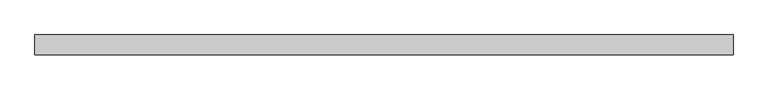
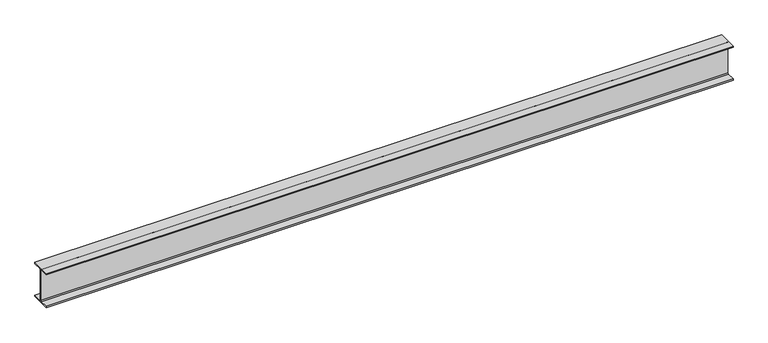
"""IFC4 building model written with IfcOpenShell, lengths in millimetres: beam geometry, Old_Steel Beam_H-KSD3502 : H_SB_ASB_H-350×175x7x11."""

import ifcopenshell
import ifcopenshell.guid

model = None  # the IFC model being written
_history = None  # IfcOwnerHistory: only IFC2X3 demands one
_inside = {}  # id of a spatial element -> (the spatial element, [elements in it])
_under = {}  # id of a project, library or spatial element -> (it, [spatial elements below it])
_declared = {}  # id of a project -> (the project, [libraries it declares])
_typed = {}  # id of a type object -> (the type object, [elements of that type])
_made_of = {}  # id of a material, layer set ... -> (it, [elements and type objects made of it])


def new_model(schema):
    """Start an empty IFC model of exactly this schema.

    Asked for "IFC4X3", IfcOpenShell would pick the latest addendum, in which some entities
    have other attributes; the version numbers below select the first issue.
    IFC2X3 requires an IfcOwnerHistory on every rooted entity: one is made here for all.
    """
    global model, _history
    if schema == "IFC4X3":
        model = ifcopenshell.file(schema_version=(4, 3, 0, 0))
    else:
        model = ifcopenshell.file(schema=schema)
    _inside.clear()
    _under.clear()
    _declared.clear()
    _typed.clear()
    _made_of.clear()
    _history = None
    if model.schema == "IFC2X3":
        org = make("IfcOrganization", Name="unknown")
        user = make(
            "IfcPersonAndOrganization",
            ThePerson=make("IfcPerson", FamilyName="unknown"),
            TheOrganization=org,
        )
        app = make(
            "IfcApplication",
            ApplicationDeveloper=org,
            Version="unknown",
            ApplicationFullName="unknown",
            ApplicationIdentifier="unknown",
        )
        _history = make(
            "IfcOwnerHistory",
            OwningUser=user,
            OwningApplication=app,
            ChangeAction="ADDED",
            CreationDate=0,
        )
    return model


def make(cls, **values):
    """One entity of the class cls with the attributes given. An attribute that is None is left unset."""
    return model.create_entity(
        cls, **{name: value for name, value in values.items() if value is not None}
    )


def rooted(cls, **values):
    """An entity with a GlobalId (a new one), such as an element, a storey or a relation."""
    return make(cls, GlobalId=ifcopenshell.guid.new(), OwnerHistory=_history, **values)


def si_unit(unit_type, name, prefix=None):
    """IfcSIUnit, for example si_unit("LENGTHUNIT", "METRE", prefix="MILLI")."""
    return make("IfcSIUnit", UnitType=unit_type, Prefix=prefix, Name=name)


def assignment(units):
    """IfcUnitAssignment: the units of a project."""
    return None if units is None else make("IfcUnitAssignment", Units=units)


def point(xyz):
    """IfcCartesianPoint."""
    return None if xyz is None else make("IfcCartesianPoint", Coordinates=xyz)


def direction(xyz):
    """IfcDirection."""
    return None if xyz is None else make("IfcDirection", DirectionRatios=xyz)


def frame(location, z_axis=None, x_axis=None):
    """IfcAxis2Placement3D, a coordinate frame: its origin and axes. An axis left out is left unset."""
    return make(
        "IfcAxis2Placement3D",
        Location=point(location),
        Axis=direction(z_axis),
        RefDirection=direction(x_axis),
    )


def frame_2d(location, x_axis=None):
    """IfcAxis2Placement2D, a coordinate frame in the plane: its origin and x axis."""
    return make(
        "IfcAxis2Placement2D", Location=point(location), RefDirection=direction(x_axis)
    )


def origin():
    """The frame at (0, 0, 0) with its axes left unset."""
    return frame((0.0, 0.0, 0.0))


def place(relative_to, where):
    """IfcLocalPlacement: puts the frame where relative to a parent placement (None: the world)."""
    return make(
        "IfcLocalPlacement", PlacementRelTo=relative_to, RelativePlacement=where
    )


def context(
    kind, dimensions, precision=None, world=None, true_north=None, identifier=None
):
    """IfcGeometricRepresentationContext, for example the 3D "Model" context."""
    return make(
        "IfcGeometricRepresentationContext",
        ContextIdentifier=identifier,
        ContextType=kind,
        CoordinateSpaceDimension=dimensions,
        Precision=precision,
        WorldCoordinateSystem=world,
        TrueNorth=true_north,
    )


def project(units=None, contexts=None):
    """IfcProject with its units and contexts."""
    return rooted(
        "IfcProject",
        Name="project",
        RepresentationContexts=contexts,
        UnitsInContext=assignment(units),
    )


def spatial(cls, under=None, at=None, **own):
    """A site, building, storey or space (cls), placed at a placement, below another one or the project."""
    s = rooted(cls, ObjectPlacement=at, **own)
    if under is not None:
        _under.setdefault(under.id(), (under, []))[1].append(s)
    return s


def polyline(points):
    """IfcPolyline through the points."""
    return make("IfcPolyline", Points=[point(p) for p in points])


def circle_curve(where, radius):
    """IfcCircle in the frame where."""
    return make("IfcCircle", Position=where, Radius=radius)


def trimmed(basis, trim1, trim2, sense, master):
    """IfcTrimmedCurve: the piece of a basis curve between two trims."""
    return make(
        "IfcTrimmedCurve",
        BasisCurve=basis,
        Trim1=trim1,
        Trim2=trim2,
        SenseAgreement=sense,
        MasterRepresentation=master,
    )


def segment(curve, same_sense, transition):
    """IfcCompositeCurveSegment."""
    return make(
        "IfcCompositeCurveSegment",
        Transition=transition,
        SameSense=same_sense,
        ParentCurve=curve,
    )


def composite_curve(segments, self_intersect=None):
    """IfcCompositeCurve: segments joined end to end."""
    return make("IfcCompositeCurve", Segments=segments, SelfIntersect=self_intersect)


def outline(outer, holes=None, kind="AREA"):
    """IfcArbitraryClosedProfileDef: a profile drawn as a closed curve; with holes, ...WithVoids."""
    if holes is None:
        return make("IfcArbitraryClosedProfileDef", ProfileType=kind, OuterCurve=outer)
    return make(
        "IfcArbitraryProfileDefWithVoids",
        ProfileType=kind,
        OuterCurve=outer,
        InnerCurves=holes,
    )


def extrude(swept, where, along, depth):
    """IfcExtrudedAreaSolid: the profile swept, set in the frame where, extruded along a direction by depth."""
    return make(
        "IfcExtrudedAreaSolid",
        SweptArea=swept,
        Position=where,
        ExtrudedDirection=direction(along),
        Depth=depth,
    )


def shape(context_of_items, identifier, shape_type, items):
    """IfcShapeRepresentation: the items that make up one representation, for example the "Body"."""
    return make(
        "IfcShapeRepresentation",
        ContextOfItems=context_of_items,
        RepresentationIdentifier=identifier,
        RepresentationType=shape_type,
        Items=items,
    )


def source(mapping_origin, context_of_items, identifier, shape_type, items):
    """IfcRepresentationMap: a shape defined once, which mapped items show again and again."""
    return make(
        "IfcRepresentationMap",
        MappingOrigin=mapping_origin,
        MappedRepresentation=shape(context_of_items, identifier, shape_type, items),
    )


def transform(
    local_origin,
    x_axis=None,
    y_axis=None,
    z_axis=None,
    scale=None,
    scale2=None,
    scale3=None,
    uniform=True,
):
    """IfcCartesianTransformationOperator3D, or its non-uniform kind. x_axis, y_axis, z_axis: its Axis1, 2, 3."""
    if uniform:
        return make(
            "IfcCartesianTransformationOperator3D",
            Axis1=direction(x_axis),
            Axis2=direction(y_axis),
            LocalOrigin=point(local_origin),
            Scale=scale,
            Axis3=direction(z_axis),
        )
    return make(
        "IfcCartesianTransformationOperator3DnonUniform",
        Axis1=direction(x_axis),
        Axis2=direction(y_axis),
        LocalOrigin=point(local_origin),
        Scale=scale,
        Axis3=direction(z_axis),
        Scale2=scale2,
        Scale3=scale3,
    )


def mapped(mapping_source, mapping_target):
    """IfcMappedItem: shows the shape of a source again, moved by a transform."""
    return make(
        "IfcMappedItem", MappingSource=mapping_source, MappingTarget=mapping_target
    )


def made_of(thing, what):
    """Note that an element or type object is made of a material, layer set ...; save() writes the relation."""
    if what is not None:
        _made_of.setdefault(what.id(), (what, []))[1].append(thing)
    return thing


def element(
    cls,
    number,
    at=None,
    inside=None,
    cuts=None,
    type_object=None,
    material=None,
    context=None,
    identifier="Body",
    shape_type=None,
    held_by="IfcProductDefinitionShape",
    body=None,
    shapes=None,
    **own,
):
    """One element of the class cls, such as IfcWall. Its Tag is "e" and its number.

    at: its placement. inside: the storey or other place that contains it. cuts: it is an
    opening in that element (IfcRelVoidsElement). A single representation is given by context,
    identifier, shape_type and body (its items); several are given by shapes. held_by: the class
    of the entity that holds the representations. save() writes the other relations.
    """
    e = rooted(cls, Tag="e%d" % number, ObjectPlacement=at, **own)
    if body is not None:
        shapes = [shape(context, identifier, shape_type, body)]
    if shapes is not None:
        e.Representation = make(held_by, Representations=shapes)
    if inside is not None:
        _inside.setdefault(inside.id(), (inside, []))[1].append(e)
    if cuts is not None:
        rooted(
            "IfcRelVoidsElement", RelatingBuildingElement=cuts, RelatedOpeningElement=e
        )
    if type_object is not None:
        _typed.setdefault(type_object.id(), (type_object, []))[1].append(e)
    return made_of(e, material)


def aggregate(whole, parts):
    """IfcRelAggregates: a whole, such as a stair, and the parts it consists of."""
    return rooted("IfcRelAggregates", RelatingObject=whole, RelatedObjects=parts)


def save(model, path):
    """Write the relations noted so far, then the file.

    IfcRelAggregates (storeys below a building ...), IfcRelContainedInSpatialStructure (elements
    in a storey), IfcRelDefinesByType, IfcRelAssociatesMaterial and IfcRelDeclares: one each for
    every whole, place, type object, material and project.
    """
    for whole, parts in _under.values():
        aggregate(whole, parts)
    for where, things in _inside.values():
        rooted(
            "IfcRelContainedInSpatialStructure",
            RelatedElements=things,
            RelatingStructure=where,
        )
    for kind, things in _typed.values():
        rooted("IfcRelDefinesByType", RelatedObjects=things, RelatingType=kind)
    for what, things in _made_of.values():
        rooted("IfcRelAssociatesMaterial", RelatedObjects=things, RelatingMaterial=what)
    for by, libraries in _declared.values():
        rooted("IfcRelDeclares", RelatingContext=by, RelatedDefinitions=libraries)
    model.write(path)


def beam_fbd36c1c(model_context):
    return source(origin(), model_context, "Body", "SweptSolid", [
        extrude(outline(composite_curve([segment(polyline([(82.5, -141.5), (82.5, -151.7), (-82.5, -151.7), (-82.5, -141.5), (-11.9, -141.5)]), True, "CONTINUOUS"), segment(trimmed(circle_curve(frame_2d((-11.9, -132.6)), 8.9), [point((-11.9, -141.5))], [point((-3.0, -132.6))], True, "CARTESIAN"), True, "CONTINUOUS"), segment(polyline([(-3.0, -132.6), (-3.0, 132.6)]), True, "CONTINUOUS"), segment(trimmed(circle_curve(frame_2d((-11.9, 132.6)), 8.9), [point((-3.0, 132.6))], [point((-11.9, 141.5))], True, "CARTESIAN"), True, "CONTINUOUS"), segment(polyline([(-11.9, 141.5), (-82.5, 141.5), (-82.5, 151.7), (82.5, 151.7), (82.5, 141.5), (11.9, 141.5)]), True, "CONTINUOUS"), segment(trimmed(circle_curve(frame_2d((11.9, 132.6)), 8.9), [point((11.9, 141.5))], [point((3.0, 132.6))], True, "CARTESIAN"), True, "CONTINUOUS"), segment(polyline([(3.0, 132.6), (3.0, -132.6)]), True, "CONTINUOUS"), segment(trimmed(circle_curve(frame_2d((11.9, -132.6)), 8.9), [point((3.0, -132.6))], [point((11.9, -141.5))], True, "CARTESIAN"), True, "CONTINUOUS"), segment(polyline([(11.9, -141.5), (82.5, -141.5)]), True, "CONTINUOUS")], self_intersect=False)), frame((-2774.336211, 0.0, 0.0), z_axis=(1.0, 0.0, 0.0), x_axis=(0.0, 1.0, 0.0)), (0.0, 0.0, 1.0), 5797.2714142),
    ])


if __name__ == "__main__":
    model = new_model("IFC4")
    model_context = context("Model", 3, world=origin())
    ifc_project = project(units=[si_unit("LENGTHUNIT", "METRE", prefix="MILLI")], contexts=[model_context])
    site = spatial("IfcSite", under=ifc_project)
    building = spatial("IfcBuilding", under=site)
    placement = place(None, origin())
    beam_shape = beam_fbd36c1c(model_context)
    element("IfcBeam", 1, ObjectType="Old_Steel Beam_H-KSD3502 : H_SB_ASB_H-350×175x7x11", at=placement, inside=building, context=model_context, shape_type="MappedRepresentation", body=[
        mapped(beam_shape, transform((0.0, 0.0, 0.0), x_axis=(1.0, 0.0, 0.0), y_axis=(0.0, 1.0, 0.0), z_axis=(0.0, 0.0, 1.0))),
    ])
    save(model, "model.ifc")

# Revit data of these elements
# Type "Old_Steel Beam_H-KSD3502 : H_SB_ASB_H-350×175x7x11"
#   Width = 17.5 cm
#   Web Thickness = 0.7 cm
#   Web Fillet = 1.4 cm
#   Warping Constant = 282290.0 cm⁶
#   Torsional Moment of Inertia = 19.4042 cm⁴
#   Torsional Modulus = 1.0 cm³
#   Section Area = 63.14 cm²
#   Plastic Modulus weak axis = 174.0 cm³
#   Plastic Modulus strong axis = 868.0 cm³
#   Perimeter = 1.36 m²/m
#   Nominal Weight = 49.60 kgf/m
#   Moment of Inertia weak axis = 984.00 cm⁴
#   Moment of Inertia strong axis = 13600.00 cm⁴
#   Height = 35.0 cm
#   Flange Thickness = 1.1 cm
#   Elastic Modulus weak axis = 112.0 cm³
#   Elastic Modulus strong axis = 775.0 cm³
#   Centroid Vertical = 17.5 cm
#   Centroid Horizontal = 8.75 cm
#   Length [instance default] = 1.5240 m
#   Structural Material [instance default] = Steel, 45-345
#   Assembly Code = ""
# Element 1 (IfcBeam, "Old_Steel Beam_H-KSD3502 : H_SB_ASB_H-350×175x7x11")
#   Structural Material = none
# Materials
#   "Steel, 45-345": class "Metal", colour RGB 189 187 185, transparency 0, Description = "Steel 345 MPa", Cost = 0
